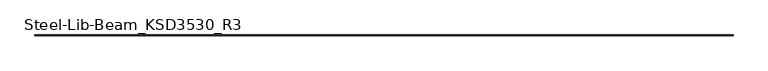
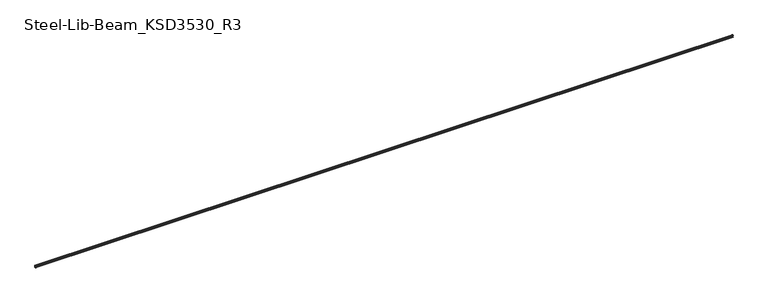
"""IFC4 building model written with IfcOpenShell, lengths in millimetres: beam geometry, Steel-Lib-Beam_KSD3530_R3 : BMS291_C-150×75x20x4.5."""

from ifc_helpers import new_model, si_unit, point, frame, frame_2d, origin, place, context, project, spatial, polyline, circle_curve, trimmed, segment, composite_curve, outline, extrude, source, transform, mapped, element, save


def steel_lib_beam_ksd3530_r3_4dedab4a(model_context):
    return source(origin(), model_context, "Body", "SweptSolid", [
        extrude(outline(composite_curve([segment(trimmed(circle_curve(frame_2d((-41.0, 66.0)), 9.0), [point((-50.0, 66.0))], [point((-41.0, 75.0))], False, "CARTESIAN"), True, "CONTINUOUS"), segment(polyline([(-41.0, 75.0), (16.0, 75.0)]), True, "CONTINUOUS"), segment(trimmed(circle_curve(frame_2d((16.0, 66.0)), 9.0), [point((16.0, 75.0))], [point((25.0, 66.0))], False, "CARTESIAN"), True, "CONTINUOUS"), segment(polyline([(25.0, 66.0), (25.0, -66.0)]), True, "CONTINUOUS"), segment(trimmed(circle_curve(frame_2d((16.0, -66.0)), 9.0), [point((25.0, -66.0))], [point((16.0, -75.0))], False, "CARTESIAN"), True, "CONTINUOUS"), segment(polyline([(16.0, -75.0), (-41.0, -75.0)]), True, "CONTINUOUS"), segment(trimmed(circle_curve(frame_2d((-41.0, -66.0)), 9.0), [point((-41.0, -75.0))], [point((-50.0, -66.0))], False, "CARTESIAN"), True, "CONTINUOUS"), segment(polyline([(-50.0, -66.0), (-50.0, -55.0), (-45.5, -55.0), (-45.5, -66.0)]), True, "CONTINUOUS"), segment(trimmed(circle_curve(frame_2d((-41.0, -66.0)), 4.5), [point((-45.5, -66.0))], [point((-41.0, -70.5))], True, "CARTESIAN"), True, "CONTINUOUS"), segment(polyline([(-41.0, -70.5), (16.0, -70.5)]), True, "CONTINUOUS"), segment(trimmed(circle_curve(frame_2d((16.0, -66.0)), 4.5), [point((16.0, -70.5))], [point((20.5, -66.0))], True, "CARTESIAN"), True, "CONTINUOUS"), segment(polyline([(20.5, -66.0), (20.5, 66.0)]), True, "CONTINUOUS"), segment(trimmed(circle_curve(frame_2d((16.0, 66.0)), 4.5), [point((20.5, 66.0))], [point((16.0, 70.5))], True, "CARTESIAN"), True, "CONTINUOUS"), segment(polyline([(16.0, 70.5), (-41.0, 70.5)]), True, "CONTINUOUS"), segment(trimmed(circle_curve(frame_2d((-41.0, 66.0)), 4.5), [point((-41.0, 70.5))], [point((-45.5, 66.0))], True, "CARTESIAN"), True, "CONTINUOUS"), segment(polyline([(-45.5, 66.0), (-45.5, 55.0), (-50.0, 55.0), (-50.0, 66.0)]), True, "CONTINUOUS")], self_intersect=False)), frame((-25664.5, 0.0, 0.0), z_axis=(1.0, 0.0, 0.0), x_axis=(0.0, 1.0, 0.0)), (0.0, 0.0, 1.0), 51329.0),
    ])


if __name__ == "__main__":
    model = new_model("IFC4")
    model_context = context("Model", 3, world=origin())
    ifc_project = project(units=[si_unit("LENGTHUNIT", "METRE", prefix="MILLI")], contexts=[model_context])
    site = spatial("IfcSite", under=ifc_project)
    building = spatial("IfcBuilding", under=site)
    placement = place(None, origin())
    steel_lib_beam_ksd3530_r3_shape = steel_lib_beam_ksd3530_r3_4dedab4a(model_context)
    element("IfcBeam", 1, ObjectType="Steel-Lib-Beam_KSD3530_R3 : BMS291_C-150×75x20x4.5", at=placement, inside=building, context=model_context, shape_type="MappedRepresentation", body=[
        mapped(steel_lib_beam_ksd3530_r3_shape, transform((0.0, 0.0, 0.0), x_axis=(1.0, 0.0, 0.0), y_axis=(0.0, 1.0, 0.0), z_axis=(0.0, 0.0, 1.0))),
    ])
    save(model, "model.ifc")

# Revit data of these elements
# Type "Steel-Lib-Beam_KSD3530_R3 : BMS291_C-150×75x20x4.5"
#   Keynote = "C-150×75x20x4.5"
#   SteelWeight = "Light"
#   x = 0.0250 m
#   t1 = 0.0090 m
#   t = 0.0045 m
#   Surface Area = 0.629834 m²/m
#   Section Area = 13.9688 cm²
#   Mass per Unit Length = 10.9655 kg/m
#   C = 0.0200 m
#   A = 0.0750 m
#   Length [instance default] = 1.5000 m
#   H = 0.1500 m
#   hec_material4 [instance default] = none
#   hec_material3 [instance default] = none
#   hec_material2 [instance default] = none
#   hec_material1 [instance default] = none
#   Structural Material [instance default] = Metal - Steel - Light Gauge
#   Assembly Code = ""
# Element 1 (IfcBeam, "Steel-Lib-Beam_KSD3530_R3 : BMS291_C-150×75x20x4.5")
#   Structural Material = none
# Materials
#   "Metal - Steel - Light Gauge": class "Metal", colour RGB 247 247 247, transparency 0
